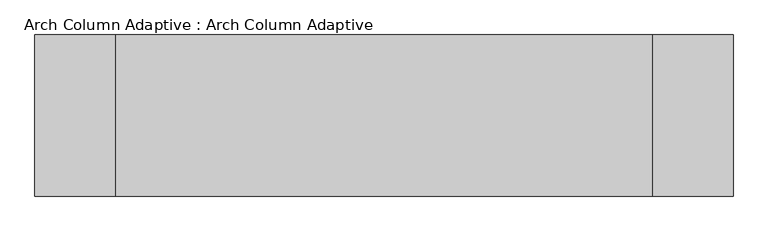
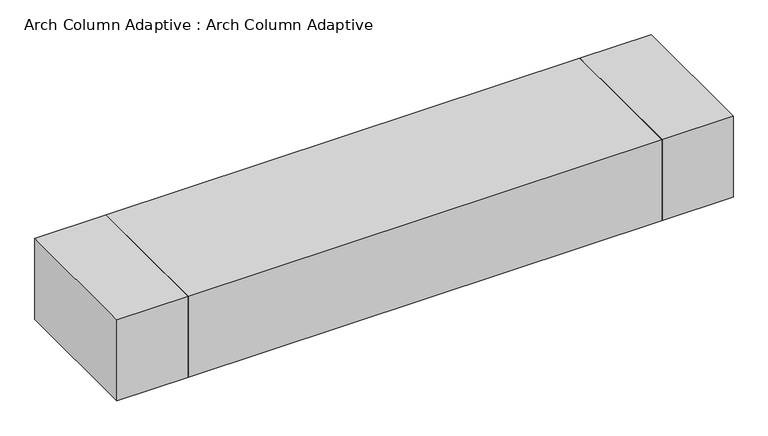
"""IFC4 building model written with IfcOpenShell, lengths in millimetres: proxy geometry, Arch Column Adaptive : Arch Column Adaptive."""

from ifc_helpers import new_model, si_unit, frame, origin, place, context, project, spatial, polyline, outline, extrude, source, transform, mapped, element, save


def arch_column_adaptive_arch_column_adaptive_969fdf9e(model_context):
    return source(origin(), model_context, "Body", "SweptSolid", [
        extrude(outline(polyline([(5000.0, -1500.0), (5000.0, 1500.0), (6500.0, 1500.0), (6500.0, -1500.0), (5000.0, -1500.0)])), frame((0.0, 0.0, 9590.0), z_axis=(0.0, 0.0, 1.0), x_axis=(1.0, 0.0, 0.0)), (0.0, 0.0, 1.0), 1800.0),
        extrude(outline(polyline([(-5000.0, 1500.0), (-5000.0, -1500.0), (-6500.0, -1500.0), (-6500.0, 1500.0), (-5000.0, 1500.0)])), frame((0.0, 0.0, 9590.0), z_axis=(0.0, 0.0, 1.0), x_axis=(1.0, 0.0, 0.0)), (0.0, 0.0, 1.0), 1800.0),
        extrude(outline(polyline([(-5000.0, -1500.0), (-5000.0, 1500.0), (5000.0, 1500.0), (5000.0, -1500.0), (-5000.0, -1500.0)])), frame((0.0, 0.0, 9590.0), z_axis=(0.0, 0.0, 1.0), x_axis=(1.0, 0.0, 0.0)), (0.0, 0.0, 1.0), 1800.0),
    ])


if __name__ == "__main__":
    model = new_model("IFC4")
    model_context = context("Model", 3, world=origin())
    ifc_project = project(units=[si_unit("LENGTHUNIT", "METRE", prefix="MILLI")], contexts=[model_context])
    site = spatial("IfcSite", under=ifc_project)
    building = spatial("IfcBuilding", under=site)
    placement = place(None, origin())
    arch_column_adaptive_arch_column_adaptive_shape = arch_column_adaptive_arch_column_adaptive_969fdf9e(model_context)
    element("IfcBuildingElementProxy", 1, Name="Arch Column Adaptive : Arch Column Adaptive", ObjectType="Arch Column Adaptive : Arch Column Adaptive", at=placement, inside=building, context=model_context, shape_type="MappedRepresentation", body=[
        mapped(arch_column_adaptive_arch_column_adaptive_shape, transform((0.0, 0.0, 0.0), x_axis=(1.0, 0.0, 0.0), y_axis=(0.0, 1.0, 0.0), z_axis=(0.0, 0.0, 1.0))),
    ])
    save(model, "model.ifc")

# Revit data of these elements
# Type "Arch Column Adaptive : Arch Column Adaptive"
#   Top Width = 3000 mm
#   Length [instance default] = 21000 mm
#   Height [instance default] = 50000 mm
#   Default Elevation = 0
# Element 1 (IfcBuildingElementProxy, "Arch Column Adaptive : Arch Column Adaptive")
#   Height = 9590 mm
